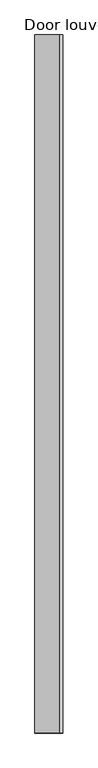
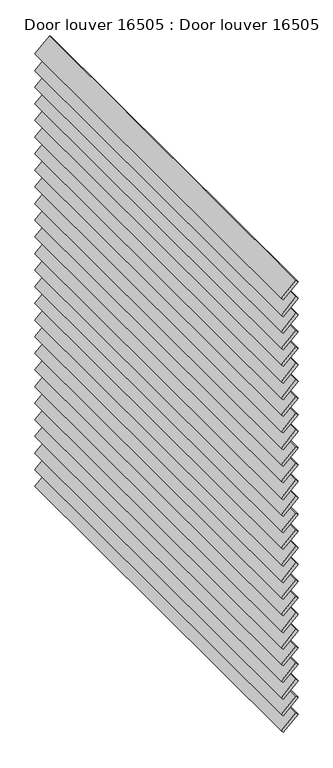
"""IFC4 building model written with IfcOpenShell, lengths in millimetres: proxy geometry, Door louver 16505 : Door louver 16505."""

from ifc_helpers import new_model, si_unit, frame, origin, place, context, project, spatial, polyline, outline, extrude, source, transform, mapped, element, save


def door_louver_16505_door_louver_16505_d946a3b7(model_context):
    return source(origin(), model_context, "Body", "SweptSolid", [
        extrude(outline(polyline([(0.0, -88.6), (0.0, 0.0), (1847.6, 0.0), (1847.6, -88.6), (0.0, -88.6)])), frame((-8304.3306423, 6540.4513244, 32854.8547367), z_axis=(-0.6925092278135618, 0.0, 0.721409016711785), x_axis=(0.0, -1.0, 0.0)), (0.0, 0.0, 1.0), 13.8216714),
        extrude(outline(polyline([(0.0, -88.6), (0.0, 0.0), (1847.6, 0.0), (1847.6, -88.6), (0.0, -88.6)])), frame((-8304.3306423, 6540.4513244, 32931.0547367), z_axis=(-0.6925092278135618, 0.0, 0.721409016711785), x_axis=(0.0, -1.0, 0.0)), (0.0, 0.0, 1.0), 13.8216714),
        extrude(outline(polyline([(0.0, -88.6), (0.0, 0.0), (1847.6, 0.0), (1847.6, -88.6), (0.0, -88.6)])), frame((-8304.3306423, 6540.4513244, 33007.2547367), z_axis=(-0.6925092278135618, 0.0, 0.721409016711785), x_axis=(0.0, -1.0, 0.0)), (0.0, 0.0, 1.0), 13.8216714),
        extrude(outline(polyline([(0.0, -88.6), (0.0, 0.0), (1847.6, 0.0), (1847.6, -88.6), (0.0, -88.6)])), frame((-8304.3306423, 6540.4513244, 33083.4547367), z_axis=(-0.6925092278135618, 0.0, 0.721409016711785), x_axis=(0.0, -1.0, 0.0)), (0.0, 0.0, 1.0), 13.8216714),
        extrude(outline(polyline([(0.0, -88.6), (0.0, 0.0), (1847.6, 0.0), (1847.6, -88.6), (0.0, -88.6)])), frame((-8304.3306423, 6540.4513244, 33159.6547367), z_axis=(-0.6925092278135618, 0.0, 0.721409016711785), x_axis=(0.0, -1.0, 0.0)), (0.0, 0.0, 1.0), 13.8216714),
        extrude(outline(polyline([(0.0, -88.6), (0.0, 0.0), (1847.6, 0.0), (1847.6, -88.6), (0.0, -88.6)])), frame((-8304.3306423, 6540.4513244, 33235.8547367), z_axis=(-0.6925092278135618, 0.0, 0.721409016711785), x_axis=(0.0, -1.0, 0.0)), (0.0, 0.0, 1.0), 13.8216714),
        extrude(outline(polyline([(0.0, -88.6), (0.0, 0.0), (1847.6, 0.0), (1847.6, -88.6), (0.0, -88.6)])), frame((-8304.3306423, 6540.4513244, 33312.0547367), z_axis=(-0.6925092278135618, 0.0, 0.721409016711785), x_axis=(0.0, -1.0, 0.0)), (0.0, 0.0, 1.0), 13.8216714),
        extrude(outline(polyline([(0.0, -88.6), (0.0, 0.0), (1847.6, 0.0), (1847.6, -88.6), (0.0, -88.6)])), frame((-8304.3306423, 6540.4513244, 33388.2547367), z_axis=(-0.6925092278135618, 0.0, 0.721409016711785), x_axis=(0.0, -1.0, 0.0)), (0.0, 0.0, 1.0), 13.8216714),
        extrude(outline(polyline([(0.0, -88.6), (0.0, 0.0), (1847.6, 0.0), (1847.6, -88.6), (0.0, -88.6)])), frame((-8304.3306423, 6540.4513244, 33464.4547367), z_axis=(-0.6925092278135618, 0.0, 0.721409016711785), x_axis=(0.0, -1.0, 0.0)), (0.0, 0.0, 1.0), 13.8216714),
        extrude(outline(polyline([(0.0, -88.6), (0.0, 0.0), (1847.6, 0.0), (1847.6, -88.6), (0.0, -88.6)])), frame((-8304.3306423, 6540.4513244, 33540.6547367), z_axis=(-0.6925092278135618, 0.0, 0.721409016711785), x_axis=(0.0, -1.0, 0.0)), (0.0, 0.0, 1.0), 13.8216714),
        extrude(outline(polyline([(0.0, -88.6), (0.0, 0.0), (1847.6, 0.0), (1847.6, -88.6), (0.0, -88.6)])), frame((-8304.3306423, 6540.4513244, 33616.8547367), z_axis=(-0.6925092278135618, 0.0, 0.721409016711785), x_axis=(0.0, -1.0, 0.0)), (0.0, 0.0, 1.0), 13.8216714),
        extrude(outline(polyline([(0.0, -88.6), (0.0, 0.0), (1847.6, 0.0), (1847.6, -88.6), (0.0, -88.6)])), frame((-8304.3306423, 6540.4513244, 33693.0547367), z_axis=(-0.6925092278135618, 0.0, 0.721409016711785), x_axis=(0.0, -1.0, 0.0)), (0.0, 0.0, 1.0), 13.8216714),
        extrude(outline(polyline([(0.0, -88.6), (0.0, 0.0), (1847.6, 0.0), (1847.6, -88.6), (0.0, -88.6)])), frame((-8304.3306423, 6540.4513244, 33769.2547367), z_axis=(-0.6925092278135618, 0.0, 0.721409016711785), x_axis=(0.0, -1.0, 0.0)), (0.0, 0.0, 1.0), 13.8216714),
        extrude(outline(polyline([(0.0, -88.6), (0.0, 0.0), (1847.6, 0.0), (1847.6, -88.6), (0.0, -88.6)])), frame((-8304.3306423, 6540.4513244, 33845.4547367), z_axis=(-0.6925092278135618, 0.0, 0.721409016711785), x_axis=(0.0, -1.0, 0.0)), (0.0, 0.0, 1.0), 13.8216714),
        extrude(outline(polyline([(0.0, -88.6), (0.0, 0.0), (1847.6, 0.0), (1847.6, -88.6), (0.0, -88.6)])), frame((-8304.3306423, 6540.4513244, 33921.6547367), z_axis=(-0.6925092278135618, 0.0, 0.721409016711785), x_axis=(0.0, -1.0, 0.0)), (0.0, 0.0, 1.0), 13.8216714),
        extrude(outline(polyline([(0.0, -88.6), (0.0, 0.0), (1847.6, 0.0), (1847.6, -88.6), (0.0, -88.6)])), frame((-8304.3306423, 6540.4513244, 33997.8547367), z_axis=(-0.6925092278135618, 0.0, 0.721409016711785), x_axis=(0.0, -1.0, 0.0)), (0.0, 0.0, 1.0), 13.8216714),
        extrude(outline(polyline([(0.0, -88.6), (0.0, 0.0), (1847.6, 0.0), (1847.6, -88.6), (0.0, -88.6)])), frame((-8304.3306423, 6540.4513244, 34074.0547367), z_axis=(-0.6925092278135618, 0.0, 0.721409016711785), x_axis=(0.0, -1.0, 0.0)), (0.0, 0.0, 1.0), 13.8216714),
        extrude(outline(polyline([(0.0, -88.6), (0.0, 0.0), (1847.6, 0.0), (1847.6, -88.6), (0.0, -88.6)])), frame((-8304.3306423, 6540.4513244, 34150.2547367), z_axis=(-0.6925092278135618, 0.0, 0.721409016711785), x_axis=(0.0, -1.0, 0.0)), (0.0, 0.0, 1.0), 13.8216714),
        extrude(outline(polyline([(0.0, -88.6), (0.0, 0.0), (1847.6, 0.0), (1847.6, -88.6), (0.0, -88.6)])), frame((-8304.3306423, 6540.4513244, 34226.4547367), z_axis=(-0.6925092278135618, 0.0, 0.721409016711785), x_axis=(0.0, -1.0, 0.0)), (0.0, 0.0, 1.0), 13.8216714),
        extrude(outline(polyline([(0.0, -88.6), (0.0, 0.0), (1847.6, 0.0), (1847.6, -88.6), (0.0, -88.6)])), frame((-8304.3306423, 6540.4513244, 34302.6547367), z_axis=(-0.6925092278135618, 0.0, 0.721409016711785), x_axis=(0.0, -1.0, 0.0)), (0.0, 0.0, 1.0), 13.8216714),
        extrude(outline(polyline([(0.0, -88.6), (0.0, 0.0), (1847.6, 0.0), (1847.6, -88.6), (0.0, -88.6)])), frame((-8304.3306423, 6540.4513244, 34378.8547367), z_axis=(-0.6925092278135618, 0.0, 0.721409016711785), x_axis=(0.0, -1.0, 0.0)), (0.0, 0.0, 1.0), 13.8216714),
        extrude(outline(polyline([(0.0, -88.6), (0.0, 0.0), (1847.6, 0.0), (1847.6, -88.6), (0.0, -88.6)])), frame((-8304.3306423, 6540.4513244, 34455.0547367), z_axis=(-0.6925092278135618, 0.0, 0.721409016711785), x_axis=(0.0, -1.0, 0.0)), (0.0, 0.0, 1.0), 13.8216714),
        extrude(outline(polyline([(0.0, -88.6), (0.0, 0.0), (1847.6, 0.0), (1847.6, -88.6), (0.0, -88.6)])), frame((-8304.3306423, 6540.4513244, 34531.2547367), z_axis=(-0.6925092278135618, 0.0, 0.721409016711785), x_axis=(0.0, -1.0, 0.0)), (0.0, 0.0, 1.0), 13.8216714),
        extrude(outline(polyline([(0.0, -88.6), (0.0, 0.0), (1847.6, 0.0), (1847.6, -88.6), (0.0, -88.6)])), frame((-8304.3306423, 6540.4513244, 34607.4547367), z_axis=(-0.6925092278135618, 0.0, 0.721409016711785), x_axis=(0.0, -1.0, 0.0)), (0.0, 0.0, 1.0), 13.8216714),
        extrude(outline(polyline([(0.0, -88.6), (0.0, 0.0), (1847.6, 0.0), (1847.6, -88.6), (0.0, -88.6)])), frame((-8304.3306423, 6540.4513244, 34683.6547367), z_axis=(-0.6925092278135618, 0.0, 0.721409016711785), x_axis=(0.0, -1.0, 0.0)), (0.0, 0.0, 1.0), 13.8216714),
        extrude(outline(polyline([(0.0, -88.6), (0.0, 0.0), (1847.6, 0.0), (1847.6, -88.6), (0.0, -88.6)])), frame((-8304.3306423, 6540.4513244, 34759.8547367), z_axis=(-0.6925092278135618, 0.0, 0.721409016711785), x_axis=(0.0, -1.0, 0.0)), (0.0, 0.0, 1.0), 13.8216714),
        extrude(outline(polyline([(0.0, -88.6), (0.0, 0.0), (1847.6, 0.0), (1847.6, -88.6), (0.0, -88.6)])), frame((-8304.3306423, 6540.4513244, 34836.0547367), z_axis=(-0.6925092278135618, 0.0, 0.721409016711785), x_axis=(0.0, -1.0, 0.0)), (0.0, 0.0, 1.0), 13.8216714),
    ])


if __name__ == "__main__":
    model = new_model("IFC4")
    model_context = context("Model", 3, world=origin())
    ifc_project = project(units=[si_unit("LENGTHUNIT", "METRE", prefix="MILLI")], contexts=[model_context])
    site = spatial("IfcSite", under=ifc_project)
    building = spatial("IfcBuilding", under=site)
    placement = place(None, origin())
    door_louver_16505_door_louver_16505_shape = door_louver_16505_door_louver_16505_d946a3b7(model_context)
    element("IfcBuildingElementProxy", 1, Name="Door louver 16505 : Door louver 16505", ObjectType="Door louver 16505 : Door louver 16505", at=placement, inside=building, context=model_context, shape_type="MappedRepresentation", body=[
        mapped(door_louver_16505_door_louver_16505_shape, transform((0.0, 0.0, 0.0), x_axis=(1.0, 0.0, 0.0), y_axis=(0.0, 1.0, 0.0), z_axis=(0.0, 0.0, 1.0))),
    ])
    save(model, "model.ifc")

# Revit data of these elements
# Type "Door louver 16505 : Door louver 16505"
#   NameOverride = "Door louver"
# Element 1 (IfcBuildingElementProxy, "Door louver 16505 : Door louver 16505")
#   Materials on its faces: "WOODEN LOUVERS (SPEC T. B. D.)"
# Materials
#   "WOODEN LOUVERS (SPEC T. B. D.)": class "Unassigned", colour RGB 148 103 60, transparency 0, Cost = 0
